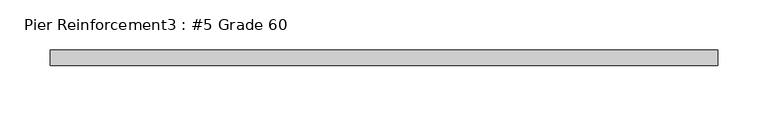
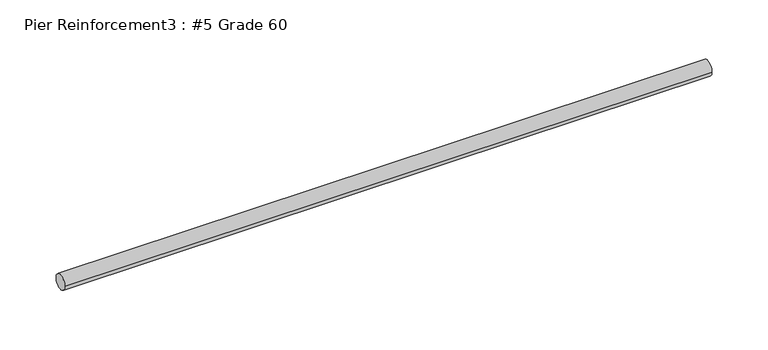
"""IFC4 building model written with IfcOpenShell, lengths in millimetres: proxy geometry, Pier Reinforcement3 : #5 Grade 60."""

from ifc_helpers import new_model, si_unit, point, frame, frame_2d, origin, place, context, project, spatial, circle_curve, trimmed, segment, composite_curve, outline, extrude, source, transform, mapped, element, save


def pier_reinforcement3_5_grade_60_c3fb3d78(model_context):
    return source(origin(), model_context, "Body", "SweptSolid", [
        extrude(outline(composite_curve([segment(trimmed(circle_curve(frame_2d((-536315.9913841, -55.5625)), 7.9375), [point((-536308.0538841, -55.5625))], [point((-536323.9288841, -55.5625))], False, "CARTESIAN"), True, "CONTINUOUS"), segment(trimmed(circle_curve(frame_2d((-536315.9913841, -55.5625)), 7.9375), [point((-536323.9288841, -55.5625))], [point((-536308.0538841, -55.5625))], False, "CARTESIAN"), True, "CONTINUOUS")], self_intersect=False)), frame((589567.2422365, 0.0, 0.0), z_axis=(1.0, 0.0, 0.0), x_axis=(0.0, 1.0, 0.0)), (0.0, 0.0, 1.0), 666.75),
    ])


if __name__ == "__main__":
    model = new_model("IFC4")
    model_context = context("Model", 3, world=origin())
    ifc_project = project(units=[si_unit("LENGTHUNIT", "METRE", prefix="MILLI")], contexts=[model_context])
    site = spatial("IfcSite", under=ifc_project)
    building = spatial("IfcBuilding", under=site)
    placement = place(None, origin())
    pier_reinforcement3_5_grade_60_shape = pier_reinforcement3_5_grade_60_c3fb3d78(model_context)
    element("IfcBuildingElementProxy", 1, Name="Pier Reinforcement3 : #5 Grade 60", ObjectType="Pier Reinforcement3 : #5 Grade 60", at=placement, inside=building, context=model_context, shape_type="MappedRepresentation", body=[
        mapped(pier_reinforcement3_5_grade_60_shape, transform((0.0, 0.0, 0.0), x_axis=(1.0, 0.0, 0.0), y_axis=(0.0, 1.0, 0.0), z_axis=(0.0, 0.0, 1.0))),
    ])
    save(model, "model.ifc")

# Revit data of these elements
# Element 1 (IfcBuildingElementProxy, "Pier Reinforcement3 : #5 Grade 60")
#   Materials on its faces: "#4 GR. 60 REINF. @ 16\" O.C. EW."
# Materials
#   "#4 GR. 60 REINF. @ 16\" O.C. EW.": class "Generic", colour RGB 84 83 81, transparency 0, Cost = 0
